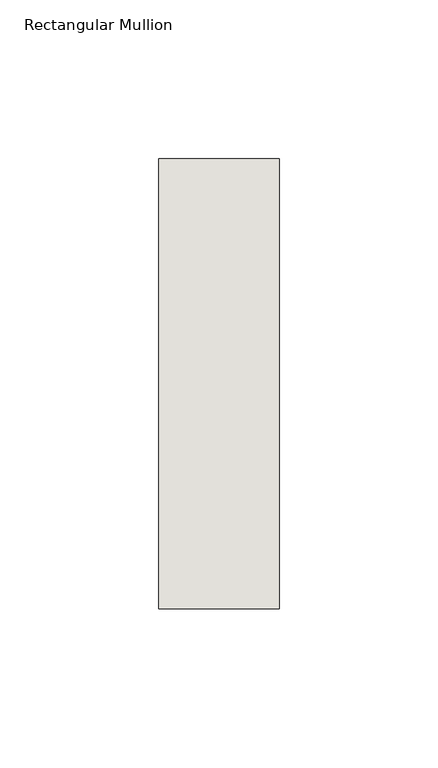
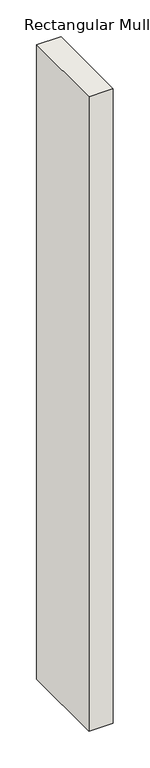
"""IFC4 building model written with IfcOpenShell, lengths in millimetres: wall geometry, Rectangular Mullion : NLRS_21_CWM_hsb-regel 38x142_gen_rsf."""

from ifc_helpers import new_model, si_unit, frame, origin, place, context, project, spatial, polyline, outline, extrude, source, transform, mapped, element, save


def rectangular_mullion_a4b8200b(model_context):
    return source(origin(), model_context, "Body", "SweptSolid", [
        extrude(outline(polyline([(0.0, -71.0), (-38.0, -71.0), (-38.0, 71.0), (0.0, 71.0), (0.0, -71.0)])), frame((0.0, 0.0, -1050.0), z_axis=(0.0, 0.0, 1.0), x_axis=(1.0, 0.0, 0.0)), (0.0, 0.0, 1.0), 1050.0),
    ])


if __name__ == "__main__":
    model = new_model("IFC4")
    model_context = context("Model", 3, world=origin())
    ifc_project = project(units=[si_unit("LENGTHUNIT", "METRE", prefix="MILLI")], contexts=[model_context])
    site = spatial("IfcSite", under=ifc_project)
    building = spatial("IfcBuilding", under=site)
    placement = place(None, origin())
    rectangular_mullion_shape = rectangular_mullion_a4b8200b(model_context)
    element("IfcWall", 1, ObjectType="Rectangular Mullion : NLRS_21_CWM_hsb-regel 38x142_gen_rsf", at=placement, inside=building, context=model_context, shape_type="MappedRepresentation", body=[
        mapped(rectangular_mullion_shape, transform((0.0, 0.0, 0.0), x_axis=(1.0, 0.0, 0.0), y_axis=(0.0, 1.0, 0.0), z_axis=(0.0, 0.0, 1.0))),
    ])
    save(model, "model.ifc")

# Revit data of these elements
# Type "Rectangular Mullion : NLRS_21_CWM_hsb-regel 38x142_gen_rsf"
#   Type IfcGUID = "07M7mRoiH1CR8m_RSKIwpF"
#   Assembly Code = "21.10"
#   IfcExportAs = "IfcWall"
#   built-in parameter 1007322 = 0.465879 (stored number, unit not read)
#   built-in parameter 1007321 = 0.062336 (stored number, unit not read)
#   built-in parameter 1007320 = 0.062336 (stored number, unit not read)
# Element 1 (IfcWall, "Rectangular Mullion : NLRS_21_CWM_hsb-regel 38x142_gen_rsf")
#   Materials on its faces: "NLRS_i2_hout naaldhout vuren_gen_rsf"
# Materials
#   "NLRS_i2_hout naaldhout vuren_gen_rsf": class "I - Hout", colour RGB 234 199 147, transparency 0, Keynote = "i2", Manufacturer = "Revit Standards Foundation", URL = "www.revitstandards.org", Description = "hout vuren", Cost = 0
